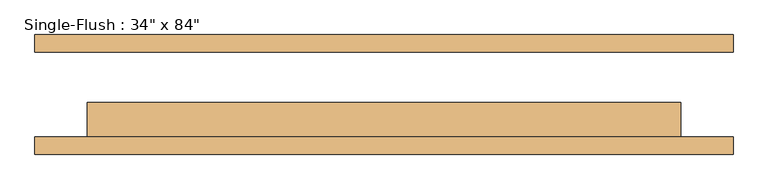
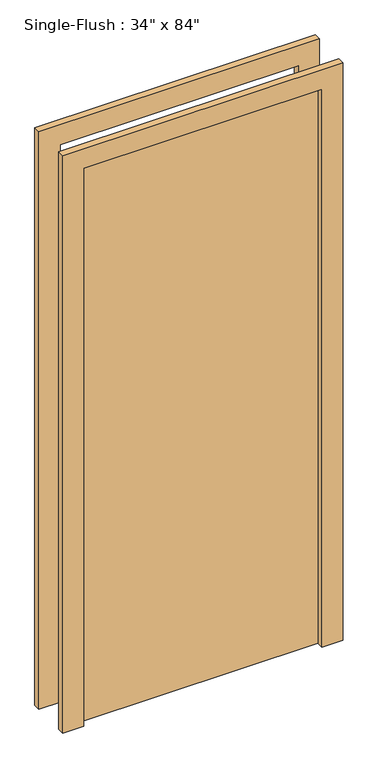
"""IFC4 building model written with IfcOpenShell, lengths in millimetres: door geometry."""

from ifc_helpers import new_model, si_unit, frame, origin, origin_with_axes, place, context, project, spatial, polyline, outline, extrude, source, transform, mapped, element, save


def door_3b0d1d25(model_context):
    return source(origin(), model_context, "Body", "SweptSolid", [
        extrude(outline(polyline([(2209.8, -508.0), (0.0, -508.0), (0.0, -431.8), (2133.6, -431.8), (2133.6, 431.8), (0.0, 431.8), (0.0, 508.0), (2209.8, 508.0), (2209.8, -508.0)])), frame((0.0, -87.3125, 0.0), z_axis=(0.0, 1.0, 0.0), x_axis=(0.0, 0.0, 1.0)), (0.0, 0.0, 1.0), 25.4),
        extrude(outline(polyline([(2209.8, 508.0), (2209.8, -508.0), (0.0, -508.0), (0.0, -431.8), (2133.6, -431.8), (2133.6, 431.8), (0.0, 431.8), (0.0, 508.0), (2209.8, 508.0)])), frame((0.0, 61.9125, 0.0), z_axis=(0.0, 1.0, 0.0), x_axis=(0.0, 0.0, 1.0)), (0.0, 0.0, 1.0), 25.4),
        extrude(outline(polyline([(431.8, -11.1125), (431.8, -61.9125), (-431.8, -61.9125), (-431.8, -11.1125), (431.8, -11.1125)])), origin_with_axes(), (0.0, 0.0, 1.0), 2133.6),
    ])


if __name__ == "__main__":
    model = new_model("IFC4")
    model_context = context("Model", 3, world=origin())
    ifc_project = project(units=[si_unit("LENGTHUNIT", "METRE", prefix="MILLI")], contexts=[model_context])
    site = spatial("IfcSite", under=ifc_project)
    building = spatial("IfcBuilding", under=site)
    placement = place(None, origin())
    door_shape = door_3b0d1d25(model_context)
    element("IfcDoor", 1, ObjectType="Single-Flush : 34\" x 84\"", at=placement, inside=building, context=model_context, shape_type="MappedRepresentation", body=[
        mapped(door_shape, transform((0.0, 0.0, 0.0), x_axis=(1.0, 0.0, 0.0), y_axis=(0.0, 1.0, 0.0), z_axis=(0.0, 0.0, 1.0))),
    ])
    save(model, "model.ifc")

# Revit data of these elements
# Type "Single-Flush : 34\" x 84\""
#   Type Mark = "2"
#   Assembly Code = "C1020"
#   Thickness = 0' - 2"
#   Height = 7' - 0"
#   Trim Projection Ext = 0' - 1"
#   Trim Projection Int = 0' - 1"
#   Trim Width = 0' - 3"
#   Width = 2' - 10"
#   Door Material = Door - Panel
#   Frame Material = Door - Frame
#   Function = (empty or 0)
#   Wall Closure = (empty or 0)
# Element 1 (IfcDoor, "Single-Flush : 34\" x 84\"")
#   Materials on its faces: "Door - Frame", "Door - Panel"
# Materials
#   "Door - Panel": class "Wood", colour RGB 114 82 51, transparency 0
#   "Door - Frame": class "Miscellaneous", colour RGB 153 76 43, transparency 0
